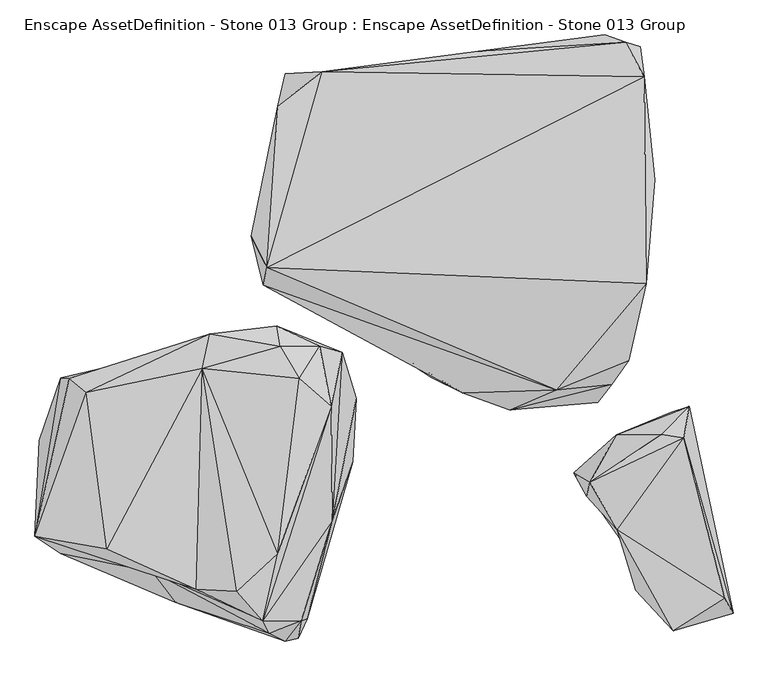
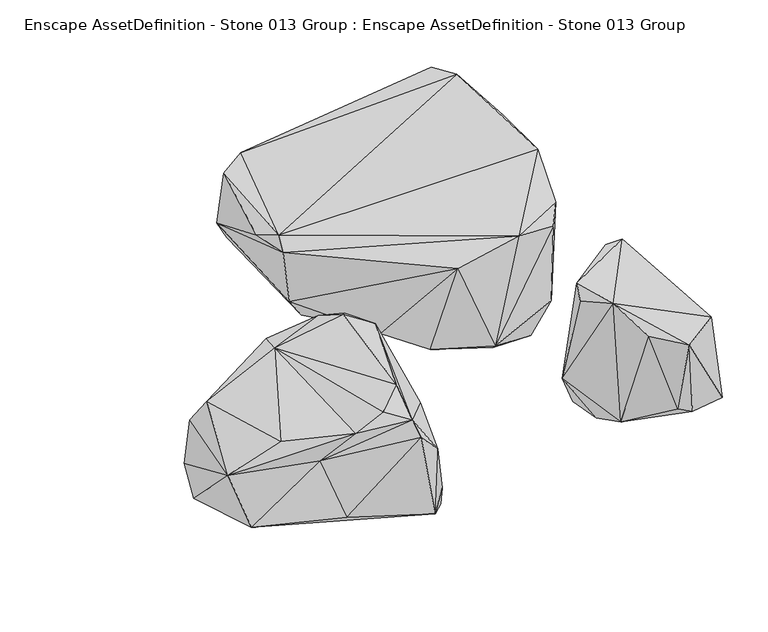
"""IFC4 building model written with IfcOpenShell, lengths in millimetres: geographic element geometry, Enscape AssetDefinition - Stone 013 Group : Enscape AssetDefinition - Stone 013 Group."""

from ifc_helpers import new_model, si_unit, origin, place, context, project, spatial, faceted_brep, source, transform, mapped, element, save


def enscape_assetdefinition_stone_013_group_enscape_1b40573f(model_context):
    return source(origin(), model_context, "Body", "Brep", [
        faceted_brep([(-441.3238168, 259.9335015, 139.7382319), (-470.200628, 250.4096329, 349.9996066), (-414.6840572, 780.6910872, 126.4466494), (30.7606645, -20.3903485, 276.044637), (264.9123371, -12.4537833, 319.1909492), (-461.001128, 294.6288586, 389.5230889), (-500.1398325, 373.9302158, 356.4640284), (-186.0505193, 108.0437899, 15.489256), (148.0788141, -63.0222708, -48.5781059), (-49.2057353, 18.7137853, -43.0800915), (-181.0707301, 199.80371, -20.1379526), (-66.2899837, 197.0043182, -43.6971672), (176.8395156, 1.0393348, -103.1484678), (403.6198854, 1.577716, 301.1038303), (369.1951334, -44.4879457, 43.4025452), (296.2891161, -36.9170196, -73.2726231), (291.3438678, 77.9635459, -136.8073523), (44.9121259, 792.434752, -9.316585), (-152.4549574, 762.9494667, -5.521046), (315.5835271, 760.0483298, -92.8952247), (330.8050036, 849.3754864, -59.2315271), (-21.3135611, 802.755177, 24.9785818), (-402.7158618, 737.3845577, 91.3117528), (-376.2209713, 295.1221466, 42.2969945), (-23.2194867, 784.2342257, 108.2712337), (-321.8607605, 785.9040499, 373.0041087), (-433.8018596, 700.1479268, 382.2103441), (70.6680492, 837.6548886, 365.5109107), (386.4780366, 878.6313534, 13.1409159), (438.8439953, 859.9358201, 401.6563594), (471.9318748, 805.8683872, 125.3343821), (476.0805964, 849.148035, 287.6721323), (485.9019816, 773.1902003, 410.1150036), (360.2537811, 797.7455854, -70.9233209), (512.4534965, 515.4131055, 394.1650689), (482.2340906, 475.777328, 94.4527909), (490.3740883, 253.8318634, 424.5716035), (447.398603, 61.4474341, 344.7088897), (382.0030391, 120.8459437, -100.3625095), (334.1811895, 159.0086222, -145.6239522)], [[[0, 1, 2]], [[1, 0, 3]], [[1, 4, 5]], [[2, 1, 6]], [[1, 3, 4]], [[6, 1, 5]], [[0, 7, 3]], [[8, 3, 9]], [[4, 3, 8]], [[7, 9, 3]], [[7, 0, 10]], [[11, 9, 7]], [[7, 10, 11]], [[11, 12, 9]], [[12, 8, 9]], [[4, 8, 13]], [[14, 13, 8]], [[12, 15, 8]], [[15, 14, 8]], [[15, 12, 16]], [[11, 16, 12]], [[16, 11, 17]], [[11, 18, 17]], [[10, 18, 11]], [[16, 17, 19]], [[17, 20, 19]], [[17, 21, 20]], [[18, 21, 17]], [[22, 18, 23]], [[10, 23, 18]], [[21, 18, 2]], [[18, 22, 2]], [[23, 0, 2]], [[23, 10, 0]], [[22, 23, 2]], [[24, 2, 25]], [[26, 2, 6]], [[25, 2, 26]], [[21, 2, 24]], [[27, 24, 25]], [[27, 21, 24]], [[28, 27, 29]], [[21, 27, 28]], [[29, 27, 25]], [[30, 28, 29]], [[30, 29, 31]], [[25, 32, 29]], [[32, 31, 29]], [[20, 21, 28]], [[30, 33, 28]], [[28, 33, 20]], [[34, 30, 31]], [[34, 35, 30]], [[35, 33, 30]], [[31, 32, 34]], [[25, 5, 32]], [[36, 32, 5]], [[36, 34, 32]], [[36, 35, 34]], [[14, 35, 37]], [[33, 35, 38]], [[38, 35, 14]], [[36, 37, 35]], [[5, 4, 36]], [[4, 37, 36]], [[5, 25, 26]], [[5, 26, 6]], [[4, 13, 37]], [[13, 14, 37]], [[16, 38, 14]], [[15, 16, 14]], [[16, 39, 38]], [[33, 38, 39]], [[16, 19, 39]], [[33, 39, 19]], [[20, 33, 19]]]),
        faceted_brep([(-433.2481027, -422.7731824, 220.9224552), (-299.7689247, -53.7440702, 193.035081), (-379.6930909, 16.2867494, 213.1471187), (-328.3635676, 97.8961289, 152.5672525), (-272.0082104, 81.3022777, 60.4570396), (-470.7591534, -592.1118259, 194.3959147), (-296.8870103, -341.941148, 51.4686666), (-622.6143241, 40.9323275, 150.7054716), (-427.4305105, 96.1802229, 177.4536967), (-536.3994837, -518.3565021, 205.2815855), (-638.4433508, -513.2864714, 152.3945034), (-913.5992527, -18.5007341, 75.238049), (-862.3571396, -411.4230275, 137.4522597), (-604.3084264, 127.3420304, 129.1807741), (-436.1914396, 147.8916705, 130.3237528), (-956.6064477, 16.4537355, -4.3886225), (-537.4704599, 121.4016005, -124.79119), (-1042.955637, -380.8178604, 45.592539), (-748.7020493, -469.9962139, 54.5502007), (-978.318274, 17.5429732, -171.4259535), (-1032.3818922, -138.9628053, -196.3344663), (-979.2549014, -423.1724143, -157.0652723), (-409.3952179, 38.7922376, -180.9047163), (-246.0526824, -193.9957291, -222.4809825), (-359.9543869, -587.6857638, -180.6715131), (-414.2982364, -643.2254314, -169.2810506), (-690.4398203, -545.7342267, -144.9608058), (-375.2977252, -592.9179192, 46.2988615), (-382.6489151, -636.2657547, -79.4894397), (-237.2619957, -33.6656161, -170.9460914), (-455.1547468, -623.5576868, 138.582781), (-257.5947642, 23.8010548, -140.3265148)], [[[0, 1, 2]], [[1, 3, 2]], [[3, 1, 4]], [[0, 5, 1]], [[1, 6, 4]], [[5, 6, 1]], [[0, 2, 7]], [[7, 2, 8]], [[2, 3, 8]], [[0, 7, 9]], [[9, 5, 0]], [[9, 7, 10]], [[10, 5, 9]], [[11, 12, 7]], [[7, 12, 10]], [[7, 8, 13]], [[13, 11, 7]], [[8, 3, 14]], [[8, 14, 13]], [[15, 13, 16]], [[14, 16, 13]], [[13, 15, 11]], [[12, 11, 17]], [[11, 15, 17]], [[12, 17, 10]], [[17, 18, 10]], [[18, 5, 10]], [[15, 19, 17]], [[17, 20, 21]], [[18, 17, 21]], [[17, 19, 20]], [[19, 15, 16]], [[19, 22, 23]], [[20, 19, 23]], [[19, 16, 22]], [[23, 24, 20]], [[21, 20, 24]], [[21, 24, 25]], [[26, 18, 21]], [[26, 21, 25]], [[24, 6, 27]], [[23, 6, 24]], [[24, 27, 28]], [[24, 28, 25]], [[23, 29, 6]], [[22, 29, 23]], [[4, 6, 29]], [[27, 6, 5]], [[27, 30, 25]], [[5, 30, 27]], [[27, 25, 28]], [[25, 30, 26]], [[18, 26, 30]], [[5, 18, 30]], [[4, 31, 14]], [[3, 4, 14]], [[31, 4, 29]], [[31, 29, 22]], [[16, 14, 31]], [[16, 31, 22]]]),
        faceted_brep([(531.5060019, -587.9477859, -115.0571406), (558.9145422, -617.5270677, 148.6431062), (464.5999372, -515.815258, 153.5701007), (582.8009844, -593.8017964, -139.6576166), (708.6488008, -573.5323429, -139.9215311), (687.8927946, -536.3841057, 165.0133431), (418.3874428, -364.1980886, 208.4840387), (429.0034473, -393.3215141, -248.7004399), (575.6523013, -276.622355, -263.8442218), (598.6846685, -54.1221835, -49.5512225), (585.2443576, -132.66249, 267.2366798), (349.0734994, -245.3223616, 243.5901463), (527.8102756, -124.6251687, 260.1523101), (414.9901569, -125.1750588, 49.0646623), (552.8070927, -69.1028088, -173.7042367), (308.4693849, -221.4253396, -138.0424649), (341.6359723, -280.4668546, 195.9102899), (399.9337256, -148.3696103, -246.7455715), (394.815743, -295.4484224, -280.2739441), (355.9256196, -208.5627317, -254.0660203)], [[[0, 1, 2]], [[3, 4, 1]], [[1, 4, 5]], [[6, 1, 5]], [[0, 3, 1]], [[2, 1, 6]], [[0, 2, 7]], [[6, 7, 2]], [[7, 3, 0]], [[4, 3, 8]], [[3, 7, 8]], [[9, 10, 4]], [[5, 4, 10]], [[4, 8, 9]], [[10, 6, 5]], [[10, 11, 6]], [[10, 12, 11]], [[12, 10, 9]], [[9, 13, 12]], [[8, 14, 9]], [[14, 13, 9]], [[13, 11, 12]], [[13, 15, 11]], [[6, 11, 16]], [[16, 11, 15]], [[17, 13, 14]], [[15, 13, 17]], [[17, 14, 8]], [[18, 17, 8]], [[19, 15, 17]], [[19, 17, 18]], [[7, 18, 8]], [[7, 15, 18]], [[18, 15, 19]], [[15, 7, 6]], [[15, 6, 16]]]),
    ])


if __name__ == "__main__":
    model = new_model("IFC4")
    model_context = context("Model", 3, world=origin())
    ifc_project = project(units=[si_unit("LENGTHUNIT", "METRE", prefix="MILLI")], contexts=[model_context])
    site = spatial("IfcSite", under=ifc_project)
    building = spatial("IfcBuilding", under=site)
    placement = place(None, origin())
    enscape_assetdefinition_stone_013_group_enscape_shape = enscape_assetdefinition_stone_013_group_enscape_1b40573f(model_context)
    element("IfcGeographicElement", 1, ObjectType="Enscape AssetDefinition - Stone 013 Group : Enscape AssetDefinition - Stone 013 Group", at=placement, inside=building, context=model_context, shape_type="MappedRepresentation", body=[
        mapped(enscape_assetdefinition_stone_013_group_enscape_shape, transform((0.0, 0.0, 0.0), x_axis=(1.0, 0.0, 0.0), y_axis=(0.0, 1.0, 0.0), z_axis=(0.0, 0.0, 1.0))),
    ])
    save(model, "model.ifc")

# Revit data of these elements
# Type "Enscape AssetDefinition - Stone 013 Group : Enscape AssetDefinition - Stone 013 Group"
#   EnscapeAssetSource = "REMOTE"
#   EnscapeAssetId = "87299a92-e72d-4c57-a2af-6c4ccf8c1dd4"
#   Height = 0.424572 m
#   EnscapeNativeAssetHeight = 0.424572 m
#   Default Elevation = 0
